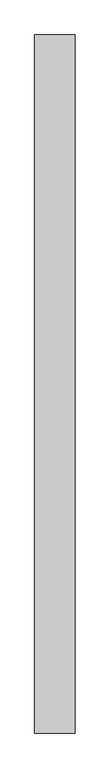
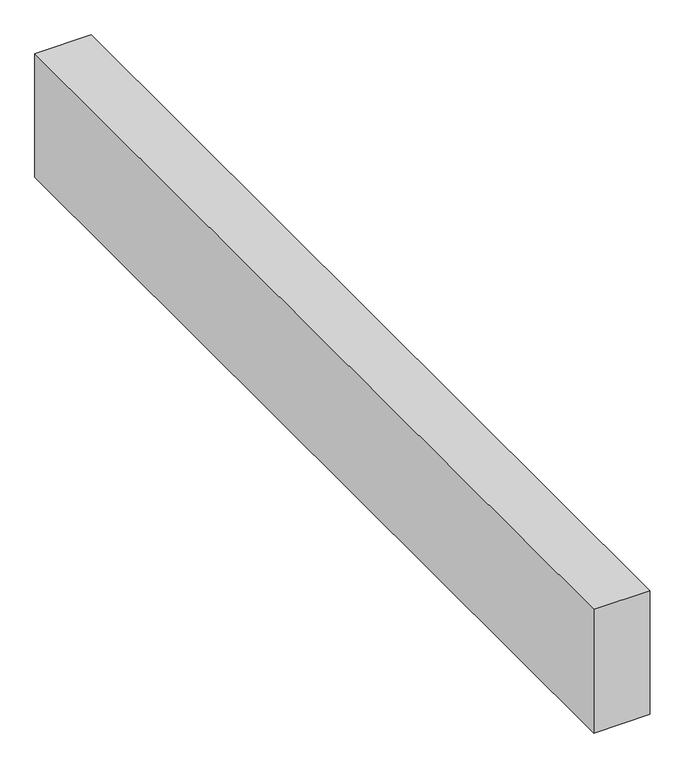
"""IFC4 building model written with IfcOpenShell, lengths in millimetres: proxy geometry, Structure002 1073 : Structure002 1073."""

from ifc_helpers import new_model, si_unit, frame, origin, place, context, project, spatial, polyline, outline, extrude, source, transform, mapped, element, save


def generic_models_3a55a6b3(model_context):
    return source(origin(), model_context, "Body", "SweptSolid", [
        extrude(outline(polyline([(5541.8883192, 7656.2019481), (5541.8883192, 10284.3743438), (5694.2883192, 10284.3743438), (5694.2883192, 7656.2019481), (5541.8883192, 7656.2019481)])), frame((0.0, 0.0, 39757.096), z_axis=(0.0, 0.0, 1.0), x_axis=(1.0, 0.0, 0.0)), (0.0, 0.0, 1.0), 355.6),
    ])


if __name__ == "__main__":
    model = new_model("IFC4")
    model_context = context("Model", 3, world=origin())
    ifc_project = project(units=[si_unit("LENGTHUNIT", "METRE", prefix="MILLI")], contexts=[model_context])
    site = spatial("IfcSite", under=ifc_project)
    building = spatial("IfcBuilding", under=site)
    placement = place(None, origin())
    generic_models_shape = generic_models_3a55a6b3(model_context)
    element("IfcBuildingElementProxy", 1, Name="Structure002 1073 : Structure002 1073", ObjectType="Structure002 1073 : Structure002 1073", at=placement, inside=building, context=model_context, shape_type="MappedRepresentation", body=[
        mapped(generic_models_shape, transform((0.0, 0.0, 0.0), x_axis=(1.0, 0.0, 0.0), y_axis=(0.0, 1.0, 0.0), z_axis=(0.0, 0.0, 1.0))),
    ])
    save(model, "model.ifc")

# Revit data of these elements
# Type "Structure002 1073 : Structure002 1073"
#   NameOverride = "Structure002"
# Element 1 (IfcBuildingElementProxy, "Structure002 1073 : Structure002 1073")
#   Materials on its faces: "STRUCTURAL MEMBER (SEE DWGS)"
# Materials
#   "STRUCTURAL MEMBER (SEE DWGS)": class "Unassigned", colour RGB 214 178 158, transparency 0, Cost = 0
